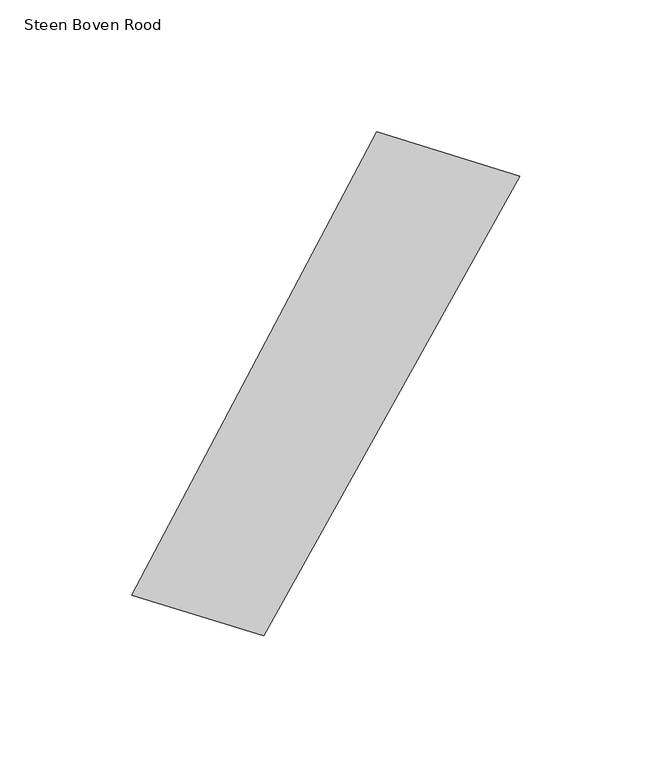
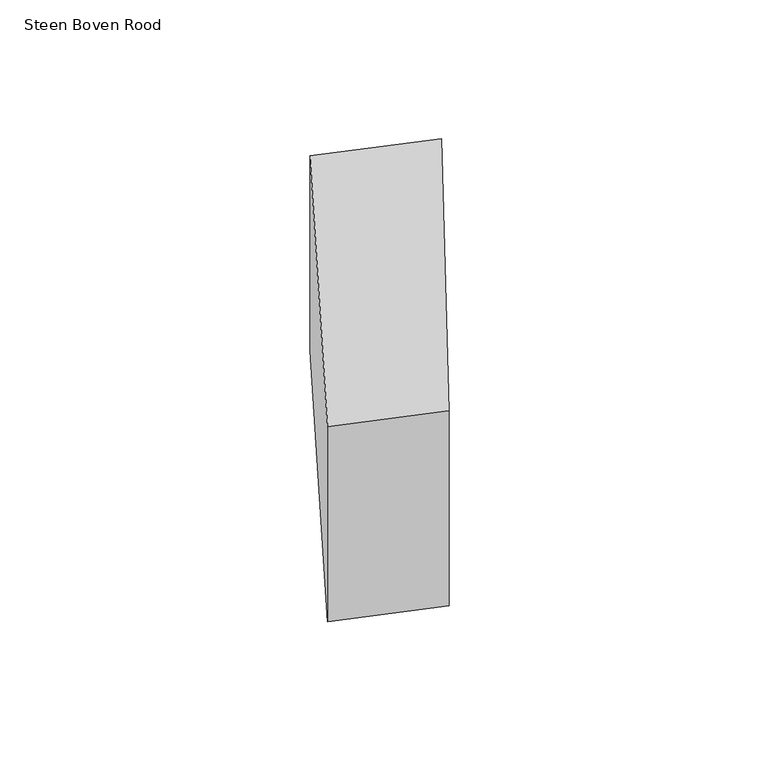
"""IFC4 building model written with IfcOpenShell, lengths in millimetres: proxy geometry, 00_GMA_steen_versie_4 : Steen Boven Rood."""

from ifc_helpers import new_model, si_unit, origin, origin_with_axes, place, context, project, spatial, polyline, outline, extrude, source, transform, mapped, element, save


def steen_boven_rood_1ffec825(model_context):
    return source(origin(), model_context, "Body", "SweptSolid", [
        extrude(outline(polyline([(150.4758943, 159.3790786), (53.5082202, -14.8628461), (3.5199999, 0.606189), (96.3363263, 176.1128255), (150.4758943, 159.3790786)])), origin_with_axes(), (0.0, 0.0, 1.0), 100.0),
    ])


if __name__ == "__main__":
    model = new_model("IFC4")
    model_context = context("Model", 3, world=origin())
    ifc_project = project(units=[si_unit("LENGTHUNIT", "METRE", prefix="MILLI")], contexts=[model_context])
    site = spatial("IfcSite", under=ifc_project)
    building = spatial("IfcBuilding", under=site)
    placement = place(None, origin())
    steen_boven_rood_shape = steen_boven_rood_1ffec825(model_context)
    element("IfcBuildingElementProxy", 1, Name="00_GMA_steen_versie_4 : Steen Boven Rood", ObjectType="00_GMA_steen_versie_4 : Steen Boven Rood", at=placement, inside=building, context=model_context, shape_type="MappedRepresentation", body=[
        mapped(steen_boven_rood_shape, transform((0.0, 0.0, 0.0), x_axis=(1.0, 0.0, 0.0), y_axis=(0.0, 1.0, 0.0), z_axis=(0.0, 0.0, 1.0))),
    ])
    save(model, "model.ifc")

# Revit data of these elements
# Type "00_GMA_steen_versie_4 : Steen Boven Rood"
#   StootVoegHalfBoven [instance default] = 5 mm
#   StootVoegHalf [instance default] = 5 mm
#   StootVoegBreedteOnder = 10 mm
#   StootVoegBreedteBoven = 10 mm
#   Steendikte = 100 mm
#   LintVoegOnderHalf = 5 mm
#   LintVoegOnder = 10 mm
#   LintVoegBovenHalf = 0 mm
#   LintVoegBoven = 0 mm
#   materiaal = 21_steen_rood
#   MateriaalVoeg = none
#   Default Elevation = 0
# Element 1 (IfcBuildingElementProxy, "00_GMA_steen_versie_4 : Steen Boven Rood")
#   Materials on its faces: "21_steen_rood"
# Materials
#   "21_steen_rood": class "Unassigned", colour RGB 213 111 43, transparency 0, Cost = 0
